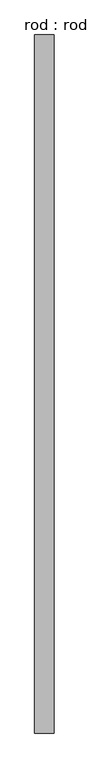
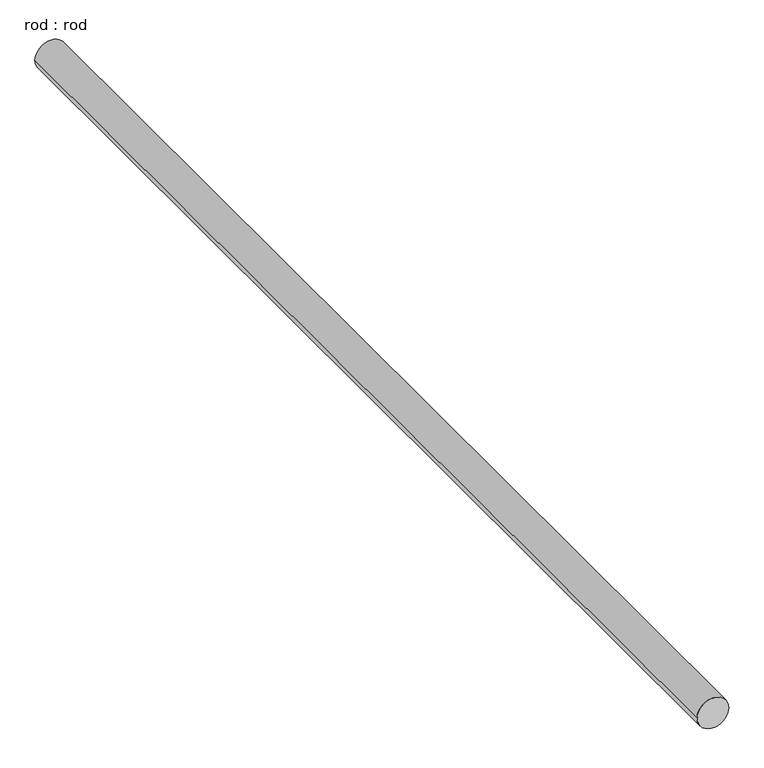
"""IFC4 building model written with IfcOpenShell, lengths in millimetres: proxy geometry, rod : rod."""

import ifcopenshell
import ifcopenshell.guid

model = None  # the IFC model being written
_history = None  # IfcOwnerHistory: only IFC2X3 demands one
_inside = {}  # id of a spatial element -> (the spatial element, [elements in it])
_under = {}  # id of a project, library or spatial element -> (it, [spatial elements below it])
_declared = {}  # id of a project -> (the project, [libraries it declares])
_typed = {}  # id of a type object -> (the type object, [elements of that type])
_made_of = {}  # id of a material, layer set ... -> (it, [elements and type objects made of it])


def new_model(schema):
    """Start an empty IFC model of exactly this schema.

    Asked for "IFC4X3", IfcOpenShell would pick the latest addendum, in which some entities
    have other attributes; the version numbers below select the first issue.
    IFC2X3 requires an IfcOwnerHistory on every rooted entity: one is made here for all.
    """
    global model, _history
    if schema == "IFC4X3":
        model = ifcopenshell.file(schema_version=(4, 3, 0, 0))
    else:
        model = ifcopenshell.file(schema=schema)
    _inside.clear()
    _under.clear()
    _declared.clear()
    _typed.clear()
    _made_of.clear()
    _history = None
    if model.schema == "IFC2X3":
        org = make("IfcOrganization", Name="unknown")
        user = make(
            "IfcPersonAndOrganization",
            ThePerson=make("IfcPerson", FamilyName="unknown"),
            TheOrganization=org,
        )
        app = make(
            "IfcApplication",
            ApplicationDeveloper=org,
            Version="unknown",
            ApplicationFullName="unknown",
            ApplicationIdentifier="unknown",
        )
        _history = make(
            "IfcOwnerHistory",
            OwningUser=user,
            OwningApplication=app,
            ChangeAction="ADDED",
            CreationDate=0,
        )
    return model


def make(cls, **values):
    """One entity of the class cls with the attributes given. An attribute that is None is left unset."""
    return model.create_entity(
        cls, **{name: value for name, value in values.items() if value is not None}
    )


def rooted(cls, **values):
    """An entity with a GlobalId (a new one), such as an element, a storey or a relation."""
    return make(cls, GlobalId=ifcopenshell.guid.new(), OwnerHistory=_history, **values)


def si_unit(unit_type, name, prefix=None):
    """IfcSIUnit, for example si_unit("LENGTHUNIT", "METRE", prefix="MILLI")."""
    return make("IfcSIUnit", UnitType=unit_type, Prefix=prefix, Name=name)


def assignment(units):
    """IfcUnitAssignment: the units of a project."""
    return None if units is None else make("IfcUnitAssignment", Units=units)


def point(xyz):
    """IfcCartesianPoint."""
    return None if xyz is None else make("IfcCartesianPoint", Coordinates=xyz)


def direction(xyz):
    """IfcDirection."""
    return None if xyz is None else make("IfcDirection", DirectionRatios=xyz)


def frame(location, z_axis=None, x_axis=None):
    """IfcAxis2Placement3D, a coordinate frame: its origin and axes. An axis left out is left unset."""
    return make(
        "IfcAxis2Placement3D",
        Location=point(location),
        Axis=direction(z_axis),
        RefDirection=direction(x_axis),
    )


def frame_2d(location, x_axis=None):
    """IfcAxis2Placement2D, a coordinate frame in the plane: its origin and x axis."""
    return make(
        "IfcAxis2Placement2D", Location=point(location), RefDirection=direction(x_axis)
    )


def origin():
    """The frame at (0, 0, 0) with its axes left unset."""
    return frame((0.0, 0.0, 0.0))


def place(relative_to, where):
    """IfcLocalPlacement: puts the frame where relative to a parent placement (None: the world)."""
    return make(
        "IfcLocalPlacement", PlacementRelTo=relative_to, RelativePlacement=where
    )


def context(
    kind, dimensions, precision=None, world=None, true_north=None, identifier=None
):
    """IfcGeometricRepresentationContext, for example the 3D "Model" context."""
    return make(
        "IfcGeometricRepresentationContext",
        ContextIdentifier=identifier,
        ContextType=kind,
        CoordinateSpaceDimension=dimensions,
        Precision=precision,
        WorldCoordinateSystem=world,
        TrueNorth=true_north,
    )


def project(units=None, contexts=None):
    """IfcProject with its units and contexts."""
    return rooted(
        "IfcProject",
        Name="project",
        RepresentationContexts=contexts,
        UnitsInContext=assignment(units),
    )


def spatial(cls, under=None, at=None, **own):
    """A site, building, storey or space (cls), placed at a placement, below another one or the project."""
    s = rooted(cls, ObjectPlacement=at, **own)
    if under is not None:
        _under.setdefault(under.id(), (under, []))[1].append(s)
    return s


def circle_curve(where, radius):
    """IfcCircle in the frame where."""
    return make("IfcCircle", Position=where, Radius=radius)


def trimmed(basis, trim1, trim2, sense, master):
    """IfcTrimmedCurve: the piece of a basis curve between two trims."""
    return make(
        "IfcTrimmedCurve",
        BasisCurve=basis,
        Trim1=trim1,
        Trim2=trim2,
        SenseAgreement=sense,
        MasterRepresentation=master,
    )


def segment(curve, same_sense, transition):
    """IfcCompositeCurveSegment."""
    return make(
        "IfcCompositeCurveSegment",
        Transition=transition,
        SameSense=same_sense,
        ParentCurve=curve,
    )


def composite_curve(segments, self_intersect=None):
    """IfcCompositeCurve: segments joined end to end."""
    return make("IfcCompositeCurve", Segments=segments, SelfIntersect=self_intersect)


def outline(outer, holes=None, kind="AREA"):
    """IfcArbitraryClosedProfileDef: a profile drawn as a closed curve; with holes, ...WithVoids."""
    if holes is None:
        return make("IfcArbitraryClosedProfileDef", ProfileType=kind, OuterCurve=outer)
    return make(
        "IfcArbitraryProfileDefWithVoids",
        ProfileType=kind,
        OuterCurve=outer,
        InnerCurves=holes,
    )


def extrude(swept, where, along, depth):
    """IfcExtrudedAreaSolid: the profile swept, set in the frame where, extruded along a direction by depth."""
    return make(
        "IfcExtrudedAreaSolid",
        SweptArea=swept,
        Position=where,
        ExtrudedDirection=direction(along),
        Depth=depth,
    )


def shape(context_of_items, identifier, shape_type, items):
    """IfcShapeRepresentation: the items that make up one representation, for example the "Body"."""
    return make(
        "IfcShapeRepresentation",
        ContextOfItems=context_of_items,
        RepresentationIdentifier=identifier,
        RepresentationType=shape_type,
        Items=items,
    )


def source(mapping_origin, context_of_items, identifier, shape_type, items):
    """IfcRepresentationMap: a shape defined once, which mapped items show again and again."""
    return make(
        "IfcRepresentationMap",
        MappingOrigin=mapping_origin,
        MappedRepresentation=shape(context_of_items, identifier, shape_type, items),
    )


def transform(
    local_origin,
    x_axis=None,
    y_axis=None,
    z_axis=None,
    scale=None,
    scale2=None,
    scale3=None,
    uniform=True,
):
    """IfcCartesianTransformationOperator3D, or its non-uniform kind. x_axis, y_axis, z_axis: its Axis1, 2, 3."""
    if uniform:
        return make(
            "IfcCartesianTransformationOperator3D",
            Axis1=direction(x_axis),
            Axis2=direction(y_axis),
            LocalOrigin=point(local_origin),
            Scale=scale,
            Axis3=direction(z_axis),
        )
    return make(
        "IfcCartesianTransformationOperator3DnonUniform",
        Axis1=direction(x_axis),
        Axis2=direction(y_axis),
        LocalOrigin=point(local_origin),
        Scale=scale,
        Axis3=direction(z_axis),
        Scale2=scale2,
        Scale3=scale3,
    )


def mapped(mapping_source, mapping_target):
    """IfcMappedItem: shows the shape of a source again, moved by a transform."""
    return make(
        "IfcMappedItem", MappingSource=mapping_source, MappingTarget=mapping_target
    )


def made_of(thing, what):
    """Note that an element or type object is made of a material, layer set ...; save() writes the relation."""
    if what is not None:
        _made_of.setdefault(what.id(), (what, []))[1].append(thing)
    return thing


def element(
    cls,
    number,
    at=None,
    inside=None,
    cuts=None,
    type_object=None,
    material=None,
    context=None,
    identifier="Body",
    shape_type=None,
    held_by="IfcProductDefinitionShape",
    body=None,
    shapes=None,
    **own,
):
    """One element of the class cls, such as IfcWall. Its Tag is "e" and its number.

    at: its placement. inside: the storey or other place that contains it. cuts: it is an
    opening in that element (IfcRelVoidsElement). A single representation is given by context,
    identifier, shape_type and body (its items); several are given by shapes. held_by: the class
    of the entity that holds the representations. save() writes the other relations.
    """
    e = rooted(cls, Tag="e%d" % number, ObjectPlacement=at, **own)
    if body is not None:
        shapes = [shape(context, identifier, shape_type, body)]
    if shapes is not None:
        e.Representation = make(held_by, Representations=shapes)
    if inside is not None:
        _inside.setdefault(inside.id(), (inside, []))[1].append(e)
    if cuts is not None:
        rooted(
            "IfcRelVoidsElement", RelatingBuildingElement=cuts, RelatedOpeningElement=e
        )
    if type_object is not None:
        _typed.setdefault(type_object.id(), (type_object, []))[1].append(e)
    return made_of(e, material)


def aggregate(whole, parts):
    """IfcRelAggregates: a whole, such as a stair, and the parts it consists of."""
    return rooted("IfcRelAggregates", RelatingObject=whole, RelatedObjects=parts)


def save(model, path):
    """Write the relations noted so far, then the file.

    IfcRelAggregates (storeys below a building ...), IfcRelContainedInSpatialStructure (elements
    in a storey), IfcRelDefinesByType, IfcRelAssociatesMaterial and IfcRelDeclares: one each for
    every whole, place, type object, material and project.
    """
    for whole, parts in _under.values():
        aggregate(whole, parts)
    for where, things in _inside.values():
        rooted(
            "IfcRelContainedInSpatialStructure",
            RelatedElements=things,
            RelatingStructure=where,
        )
    for kind, things in _typed.values():
        rooted("IfcRelDefinesByType", RelatedObjects=things, RelatingType=kind)
    for what, things in _made_of.values():
        rooted("IfcRelAssociatesMaterial", RelatedObjects=things, RelatingMaterial=what)
    for by, libraries in _declared.values():
        rooted("IfcRelDeclares", RelatingContext=by, RelatedDefinitions=libraries)
    model.write(path)


def rod_rod_731dede8(model_context):
    return source(origin(), model_context, "Body", "SweptSolid", [
        extrude(outline(composite_curve([segment(trimmed(circle_curve(frame_2d((0.0108462, 0.0)), 200.0), [point((0.0108462, 200.0))], [point((0.0108462, -200.0))], False, "CARTESIAN"), True, "CONTINUOUS"), segment(trimmed(circle_curve(frame_2d((0.0108462, 0.0)), 200.0), [point((0.0108462, -200.0))], [point((0.0108462, 200.0))], False, "CARTESIAN"), True, "CONTINUOUS")], self_intersect=False)), frame((0.0, -3167.7276518, 0.0), z_axis=(0.0, 1.0, 0.0), x_axis=(0.0, 0.0, 1.0)), (0.0, 0.0, 1.0), 14520.9125342),
    ])


if __name__ == "__main__":
    model = new_model("IFC4")
    model_context = context("Model", 3, world=origin())
    ifc_project = project(units=[si_unit("LENGTHUNIT", "METRE", prefix="MILLI")], contexts=[model_context])
    site = spatial("IfcSite", under=ifc_project)
    building = spatial("IfcBuilding", under=site)
    placement = place(None, origin())
    rod_rod_shape = rod_rod_731dede8(model_context)
    element("IfcBuildingElementProxy", 1, Name="rod : rod", ObjectType="rod : rod", at=placement, inside=building, context=model_context, shape_type="MappedRepresentation", body=[
        mapped(rod_rod_shape, transform((0.0, 0.0, 0.0), x_axis=(1.0, 0.0, 0.0), y_axis=(0.0, 1.0, 0.0), z_axis=(0.0, 0.0, 1.0))),
    ])
    save(model, "model.ifc")

# Revit data of these elements
# Type "rod : rod"
#   Default Elevation = 0
